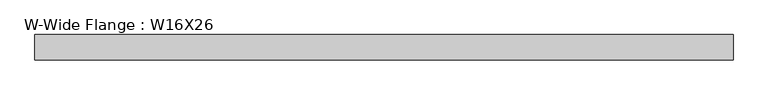
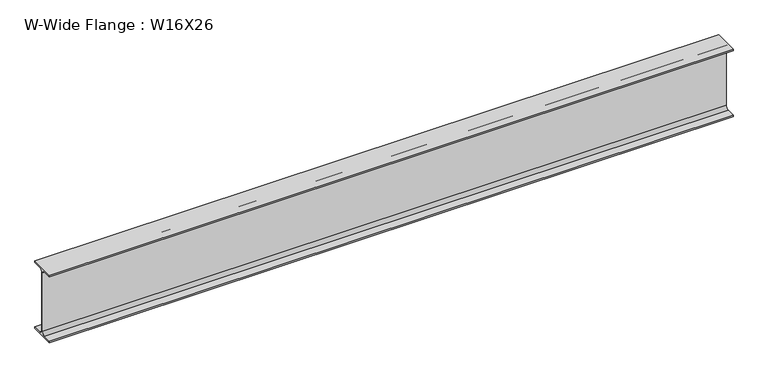
"""IFC4 building model written with IfcOpenShell, lengths in millimetres: beam geometry, W-Wide Flange : W16X26."""

from ifc_helpers import new_model, si_unit, point, frame, frame_2d, origin, place, context, project, spatial, polyline, circle_curve, trimmed, segment, composite_curve, outline, extrude, source, transform, mapped, element, save


def w_wide_flange_w16x26_7a111733(model_context):
    return source(origin(), model_context, "Body", "SweptSolid", [
        extrude(outline(composite_curve([segment(polyline([(69.85, -190.627), (69.85, -199.39), (-69.85, -199.39), (-69.85, -190.627), (-21.3995, -190.627)]), True, "CONTINUOUS"), segment(trimmed(circle_curve(frame_2d((-21.3995, -172.4025)), 18.2245), [point((-21.3995, -190.627))], [point((-3.175, -172.4025))], True, "CARTESIAN"), True, "CONTINUOUS"), segment(polyline([(-3.175, -172.4025), (-3.175, 172.4025)]), True, "CONTINUOUS"), segment(trimmed(circle_curve(frame_2d((-21.3995, 172.4025)), 18.2245), [point((-3.175, 172.4025))], [point((-21.3995, 190.627))], True, "CARTESIAN"), True, "CONTINUOUS"), segment(polyline([(-21.3995, 190.627), (-69.85, 190.627), (-69.85, 199.39), (69.85, 199.39), (69.85, 190.627), (21.3995, 190.627)]), True, "CONTINUOUS"), segment(trimmed(circle_curve(frame_2d((21.3995, 172.4025)), 18.2245), [point((21.3995, 190.627))], [point((3.175, 172.4025))], True, "CARTESIAN"), True, "CONTINUOUS"), segment(polyline([(3.175, 172.4025), (3.175, -172.4025)]), True, "CONTINUOUS"), segment(trimmed(circle_curve(frame_2d((21.3995, -172.4025)), 18.2245), [point((3.175, -172.4025))], [point((21.3995, -190.627))], True, "CARTESIAN"), True, "CONTINUOUS"), segment(polyline([(21.3995, -190.627), (69.85, -190.627)]), True, "CONTINUOUS")], self_intersect=False)), frame((-1911.35, 0.0, 0.0), z_axis=(1.0, 0.0, 0.0), x_axis=(0.0, 1.0, 0.0)), (0.0, 0.0, 1.0), 3816.35),
    ])


if __name__ == "__main__":
    model = new_model("IFC4")
    model_context = context("Model", 3, world=origin())
    ifc_project = project(units=[si_unit("LENGTHUNIT", "METRE", prefix="MILLI")], contexts=[model_context])
    site = spatial("IfcSite", under=ifc_project)
    building = spatial("IfcBuilding", under=site)
    placement = place(None, origin())
    w_wide_flange_w16x26_shape = w_wide_flange_w16x26_7a111733(model_context)
    element("IfcBeam", 1, ObjectType="W-Wide Flange : W16X26", at=placement, inside=building, context=model_context, shape_type="MappedRepresentation", body=[
        mapped(w_wide_flange_w16x26_shape, transform((0.0, 0.0, 0.0), x_axis=(1.0, 0.0, 0.0), y_axis=(0.0, 1.0, 0.0), z_axis=(0.0, 0.0, 1.0))),
    ])
    save(model, "model.ifc")

# Revit data of these elements
# Type "W-Wide Flange : W16X26"
#   Assembly Code = "B10"
#   W = 26
#   Length [instance default] = 5' - 0"
#   bf = 0' - 5 1/2"
#   d = 1' - 3.7"
#   k = 0' - 1 1/16"
#   k2 = 0' - 0.7175"
#   tf = 0' - 0.345"
#   tw = 0' - 0 1/4"
#   A = 0.0533333 SF
#   Structural Material [instance default] = Steel ASTM A992
# Element 1 (IfcBeam, "W-Wide Flange : W16X26")
#   Structural Material = Steel ASTM A36
#   Materials on its faces: "Steel ASTM A36"
# Materials
#   "Steel ASTM A992": class "Metal", colour RGB 199 199 199, transparency 0, Description = "Structural steel 50ksi", Cost = 0
#   "Steel ASTM A36": class "Metal", colour RGB 199 199 199, transparency 0, Description = "Structural steel, ASTM A36 Grade B, mill finish", Cost = 0
